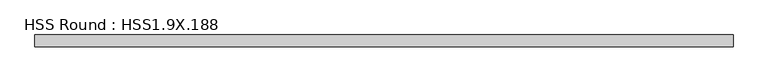
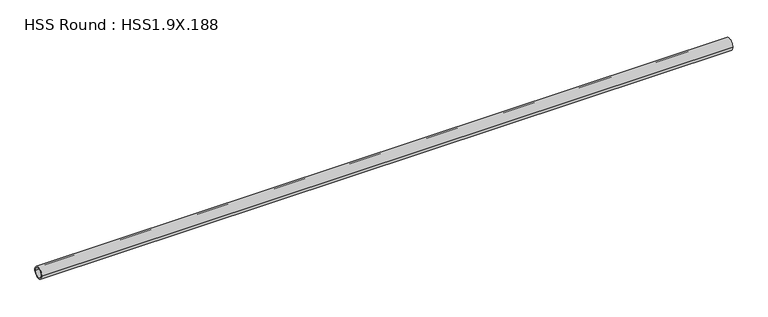
"""IFC4 building model written with IfcOpenShell, lengths in millimetres: member geometry, HSS Round : HSS1.9X.188."""

from ifc_helpers import new_model, si_unit, point, frame, origin, origin_2d, place, context, project, spatial, circle_curve, trimmed, segment, composite_curve, outline, extrude, source, transform, mapped, element, save


def hss_round_hss1_9x_188_773ecf34(model_context):
    return source(origin(), model_context, "Body", "SweptSolid", [
        extrude(outline(composite_curve([segment(trimmed(circle_curve(origin_2d(), 24.13), [point((-24.13, 0.0))], [point((24.13, 0.0))], False, "CARTESIAN"), True, "CONTINUOUS"), segment(trimmed(circle_curve(origin_2d(), 24.13), [point((24.13, 0.0))], [point((-24.13, 0.0))], False, "CARTESIAN"), True, "CONTINUOUS")], self_intersect=False), holes=[composite_curve([segment(trimmed(circle_curve(origin_2d(), 19.3548), [point((19.3548, 0.0))], [point((-19.3548, 0.0))], True, "CARTESIAN"), True, "CONTINUOUS"), segment(trimmed(circle_curve(origin_2d(), 19.3548), [point((-19.3548, 0.0))], [point((19.3548, 0.0))], True, "CARTESIAN"), True, "CONTINUOUS")], self_intersect=False)]), frame((-1473.3033114, 0.0, 0.0), z_axis=(1.0, 0.0, 0.0), x_axis=(0.0, 1.0, 0.0)), (0.0, 0.0, 1.0), 2847.6097368),
    ])


if __name__ == "__main__":
    model = new_model("IFC4")
    model_context = context("Model", 3, world=origin())
    ifc_project = project(units=[si_unit("LENGTHUNIT", "METRE", prefix="MILLI")], contexts=[model_context])
    site = spatial("IfcSite", under=ifc_project)
    building = spatial("IfcBuilding", under=site)
    placement = place(None, origin())
    hss_round_hss1_9x_188_shape = hss_round_hss1_9x_188_773ecf34(model_context)
    element("IfcMember", 1, ObjectType="HSS Round : HSS1.9X.188", at=placement, inside=building, context=model_context, shape_type="MappedRepresentation", body=[
        mapped(hss_round_hss1_9x_188_shape, transform((0.0, 0.0, 0.0), x_axis=(1.0, 0.0, 0.0), y_axis=(0.0, 1.0, 0.0), z_axis=(0.0, 0.0, 1.0))),
    ])
    save(model, "model.ifc")

# Revit data of these elements
# Type "HSS Round : HSS1.9X.188"
#   Section Name Key = "HSSRound 1.900x0.188"
#   Assembly Code = "B10"
#   Wall Nominal Thickness = 0.188"
#   Wall Design Thickness = 0.174"
#   Torsional Moment of Inertia = 0.71 in⁴
#   Torsional Modulus = 0.747 in³
#   Section Area = 0.943 in²
#   Plastic Modulus weak axis = 0.52 in³
#   Plastic Modulus strong axis = 0.52 in³
#   Nominal Weight = 3.44 lbf/ft
#   Moment of Inertia weak axis = 0.355 in⁴
#   Moment of Inertia strong axis = 0.355 in⁴
#   Elastic Modulus weak axis = 0.374 in³
#   Elastic Modulus strong axis = 0.374 in³
#   Diameter = 1.900"
#   Centroid Vertical = 0.950"
#   Centroid Horizontal = 0.950"
#   Length [instance default] = 5' - 0"
#   Structural Material [instance default] = Steel ASTM A500, Grade B, Round
#   Warping Constant = (empty or 0)
#   Principal Axes Angle = 0
# Element 1 (IfcMember, "HSS Round : HSS1.9X.188")
#   Structural Material = Steel ASTM A992
#   Materials on its faces: "Steel ASTM A992"
# Materials
#   "Steel ASTM A500, Grade B, Round": class "Metal", colour RGB 199 199 199, transparency 0, Description = "Carbon steel", Cost = 0
#   "Steel ASTM A992": class "Metal", colour RGB 199 199 199, transparency 0, Description = "Structural steel 50ksi", Cost = 0
